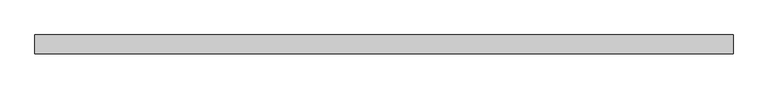
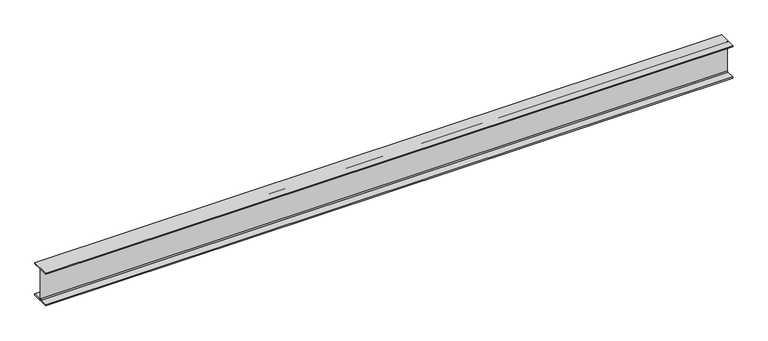
"""IFC4 building model written with IfcOpenShell, lengths in millimetres: beam geometry, Old_Steel Beam_H-KSD3502 : H_SB_ASB_H-200×200x8x12."""

from ifc_helpers import new_model, si_unit, point, frame, frame_2d, origin, place, context, project, spatial, polyline, circle_curve, trimmed, segment, composite_curve, outline, extrude, source, transform, mapped, element, save


def beam_6a3b6afb(model_context):
    return source(origin(), model_context, "Body", "SweptSolid", [
        extrude(outline(composite_curve([segment(polyline([(82.5, -141.5), (82.5, -151.7), (-82.5, -151.7), (-82.5, -141.5), (-11.9, -141.5)]), True, "CONTINUOUS"), segment(trimmed(circle_curve(frame_2d((-11.9, -132.6)), 8.9), [point((-11.9, -141.5))], [point((-3.0, -132.6))], True, "CARTESIAN"), True, "CONTINUOUS"), segment(polyline([(-3.0, -132.6), (-3.0, 132.6)]), True, "CONTINUOUS"), segment(trimmed(circle_curve(frame_2d((-11.9, 132.6)), 8.9), [point((-3.0, 132.6))], [point((-11.9, 141.5))], True, "CARTESIAN"), True, "CONTINUOUS"), segment(polyline([(-11.9, 141.5), (-82.5, 141.5), (-82.5, 151.7), (82.5, 151.7), (82.5, 141.5), (11.9, 141.5)]), True, "CONTINUOUS"), segment(trimmed(circle_curve(frame_2d((11.9, 132.6)), 8.9), [point((11.9, 141.5))], [point((3.0, 132.6))], True, "CARTESIAN"), True, "CONTINUOUS"), segment(polyline([(3.0, 132.6), (3.0, -132.6)]), True, "CONTINUOUS"), segment(trimmed(circle_curve(frame_2d((11.9, -132.6)), 8.9), [point((3.0, -132.6))], [point((11.9, -141.5))], True, "CARTESIAN"), True, "CONTINUOUS"), segment(polyline([(11.9, -141.5), (82.5, -141.5)]), True, "CONTINUOUS")], self_intersect=False)), frame((-3052.6488422, 0.0, 0.0), z_axis=(1.0, 0.0, 0.0), x_axis=(0.0, 1.0, 0.0)), (0.0, 0.0, 1.0), 6075.0680162),
    ])


if __name__ == "__main__":
    model = new_model("IFC4")
    model_context = context("Model", 3, world=origin())
    ifc_project = project(units=[si_unit("LENGTHUNIT", "METRE", prefix="MILLI")], contexts=[model_context])
    site = spatial("IfcSite", under=ifc_project)
    building = spatial("IfcBuilding", under=site)
    placement = place(None, origin())
    beam_shape = beam_6a3b6afb(model_context)
    element("IfcBeam", 1, ObjectType="Old_Steel Beam_H-KSD3502 : H_SB_ASB_H-200×200x8x12", at=placement, inside=building, context=model_context, shape_type="MappedRepresentation", body=[
        mapped(beam_shape, transform((0.0, 0.0, 0.0), x_axis=(1.0, 0.0, 0.0), y_axis=(0.0, 1.0, 0.0), z_axis=(0.0, 0.0, 1.0))),
    ])
    save(model, "model.ifc")

# Revit data of these elements
# Type "Old_Steel Beam_H-KSD3502 : H_SB_ASB_H-200×200x8x12"
#   Width = 20.0 cm
#   Web Thickness = 0.8 cm
#   Web Fillet = 1.3 cm
#   Warping Constant = 141376.0 cm⁶
#   Torsional Moment of Inertia = 26.2485 cm⁴
#   Torsional Modulus = 1.0 cm³
#   Section Area = 63.53 cm²
#   Plastic Modulus weak axis = 244.0 cm³
#   Plastic Modulus strong axis = 525.0 cm³
#   Perimeter = 1.16 m²/m
#   Nominal Weight = 49.90 kgf/m
#   Moment of Inertia weak axis = 1600.00 cm⁴
#   Moment of Inertia strong axis = 4720.00 cm⁴
#   Height = 20.0 cm
#   Flange Thickness = 1.2 cm
#   Elastic Modulus weak axis = 160.0 cm³
#   Elastic Modulus strong axis = 472.0 cm³
#   Centroid Vertical = 10.0 cm
#   Centroid Horizontal = 10.0 cm
#   Length [instance default] = 1.5240 m
#   Structural Material [instance default] = Steel, 45-345
#   Assembly Code = ""
# Element 1 (IfcBeam, "Old_Steel Beam_H-KSD3502 : H_SB_ASB_H-200×200x8x12")
#   Structural Material = none
# Materials
#   "Steel, 45-345": class "Metal", colour RGB 189 187 185, transparency 0, Description = "Steel 345 MPa", Cost = 0
